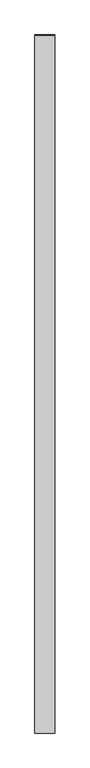
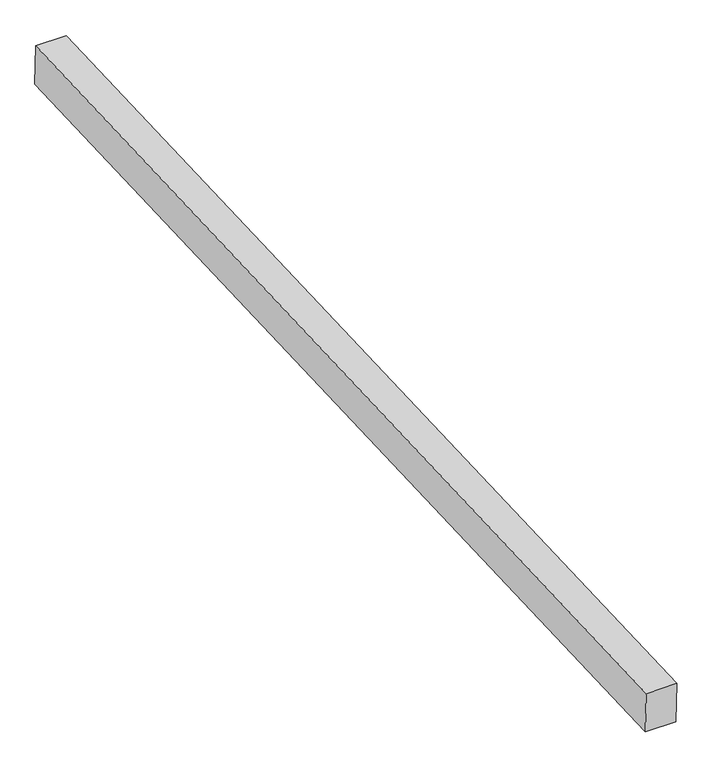
"""IFC4 building model written with IfcOpenShell, lengths in millimetres: proxy geometry, Generic Models 7:Generic Models 1:8:Generic Models 1:8 : Generic Models 7:Generic Models 1:337419:52 : Generic Models 7:Generic Models 1:8:Generic Models 1:8 : Generic Models 7:Generic Models 1:337419:315935."""

from ifc_helpers import new_model, si_unit, frame, origin, place, context, project, spatial, polyline, outline, extrude, source, transform, mapped, element, save


def generic_models_a86ed36b(model_context):
    return source(origin(), model_context, "Body", "SweptSolid", [
        extrude(outline(polyline([(-581229.2495411, 3818.908703), (-576356.3266468, 4021.9471569), (-576348.7597251, 3831.5971524), (-581221.3189223, 3628.5738526), (-581229.2495411, 3818.908703)])), frame((609597.211724, 0.0, 0.0), z_axis=(1.0, 0.0, 0.0), x_axis=(0.0, 1.0, 0.0)), (0.0, 0.0, 1.0), 139.7),
    ])


if __name__ == "__main__":
    model = new_model("IFC4")
    model_context = context("Model", 3, world=origin())
    ifc_project = project(units=[si_unit("LENGTHUNIT", "METRE", prefix="MILLI")], contexts=[model_context])
    site = spatial("IfcSite", under=ifc_project)
    building = spatial("IfcBuilding", under=site)
    placement = place(None, origin())
    generic_models_shape = generic_models_a86ed36b(model_context)
    element("IfcBuildingElementProxy", 1, Name="Generic Models 7:Generic Models 1:8:Generic Models 1:8 : Generic Models 7:Generic Models 1:337419:52 : Generic Models 7:Generic Models 1:8:Generic Models 1:8 : Generic Models 7:Generic Models 1:337419:315935", ObjectType="Generic Models 7:Generic Models 1:8:Generic Models 1:8 : Generic Models 7:Generic Models 1:337419:52 : Generic Models 7:Generic Models 1:8:Generic Models 1:8 : Generic Models 7:Generic Models 1:337419:315935", at=placement, inside=building, context=model_context, shape_type="MappedRepresentation", body=[
        mapped(generic_models_shape, transform((0.0, 0.0, 0.0), x_axis=(1.0, 0.0, 0.0), y_axis=(0.0, 1.0, 0.0), z_axis=(0.0, 0.0, 1.0))),
    ])
    save(model, "model.ifc")

# Revit data of these elements
# Type "Generic Models 7:Generic Models 1:8:Generic Models 1:8 : Generic Models 7:Generic Models 1:337419:52 : Generic Models 7:Generic Models 1:8:Generic Models 1:8 : Generic Models 7:Generic Models 1:337419:315935"
#   NameOverride = "Generic Models 7:Generic Models 1:8:Generic Models 1:8 : Generic Models 7:Generic Models 1:337419:315935"
#   ObjectTypeOverride = "Generic Models 1:8 : Generic Models 7:Generic Models 1:337419"
#   Reference = "Generic Models 1"
#   Tag = "315935"
# Element 1 (IfcBuildingElementProxy, "Generic Models 7:Generic Models 1:8:Generic Models 1:8 : Generic Models 7:Generic Models 1:337419:52 : Generic Models 7:Generic Models 1:8:Generic Models 1:8 : Generic Models 7:Generic Models 1:337419:315935")
#   Materials on its faces: "5 1/2\" X 7 1/2\" EXTERIOR GRADE GLULAM BEAMS"
# Materials
#   "5 1/2\" X 7 1/2\" EXTERIOR GRADE GLULAM BEAMS": class "Wood", colour RGB 183 134 68, transparency 0, Keynote = "M06181300.01", Description = "Pinus Echinata", Cost = 0
